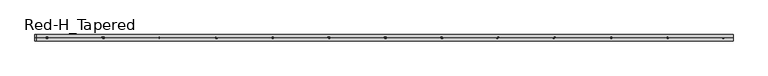
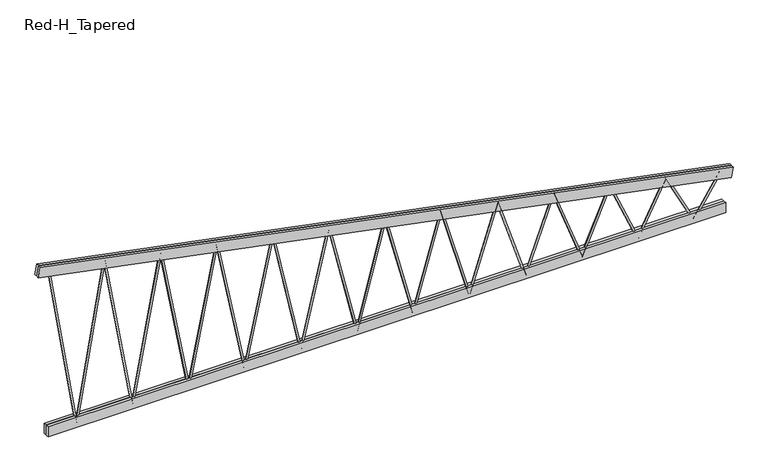
"""IFC4 building model written with IfcOpenShell, lengths in millimetres: beam geometry, Construction_Frames_RedBuilt_Openweb_Red-H_Tapered : Red-H_Tapered."""

import ifcopenshell
import ifcopenshell.guid

model = None  # the IFC model being written
_history = None  # IfcOwnerHistory: only IFC2X3 demands one
_inside = {}  # id of a spatial element -> (the spatial element, [elements in it])
_under = {}  # id of a project, library or spatial element -> (it, [spatial elements below it])
_declared = {}  # id of a project -> (the project, [libraries it declares])
_typed = {}  # id of a type object -> (the type object, [elements of that type])
_made_of = {}  # id of a material, layer set ... -> (it, [elements and type objects made of it])


def new_model(schema):
    """Start an empty IFC model of exactly this schema.

    Asked for "IFC4X3", IfcOpenShell would pick the latest addendum, in which some entities
    have other attributes; the version numbers below select the first issue.
    IFC2X3 requires an IfcOwnerHistory on every rooted entity: one is made here for all.
    """
    global model, _history
    if schema == "IFC4X3":
        model = ifcopenshell.file(schema_version=(4, 3, 0, 0))
    else:
        model = ifcopenshell.file(schema=schema)
    _inside.clear()
    _under.clear()
    _declared.clear()
    _typed.clear()
    _made_of.clear()
    _history = None
    if model.schema == "IFC2X3":
        org = make("IfcOrganization", Name="unknown")
        user = make(
            "IfcPersonAndOrganization",
            ThePerson=make("IfcPerson", FamilyName="unknown"),
            TheOrganization=org,
        )
        app = make(
            "IfcApplication",
            ApplicationDeveloper=org,
            Version="unknown",
            ApplicationFullName="unknown",
            ApplicationIdentifier="unknown",
        )
        _history = make(
            "IfcOwnerHistory",
            OwningUser=user,
            OwningApplication=app,
            ChangeAction="ADDED",
            CreationDate=0,
        )
    return model


def make(cls, **values):
    """One entity of the class cls with the attributes given. An attribute that is None is left unset."""
    return model.create_entity(
        cls, **{name: value for name, value in values.items() if value is not None}
    )


def rooted(cls, **values):
    """An entity with a GlobalId (a new one), such as an element, a storey or a relation."""
    return make(cls, GlobalId=ifcopenshell.guid.new(), OwnerHistory=_history, **values)


def si_unit(unit_type, name, prefix=None):
    """IfcSIUnit, for example si_unit("LENGTHUNIT", "METRE", prefix="MILLI")."""
    return make("IfcSIUnit", UnitType=unit_type, Prefix=prefix, Name=name)


def assignment(units):
    """IfcUnitAssignment: the units of a project."""
    return None if units is None else make("IfcUnitAssignment", Units=units)


def point(xyz):
    """IfcCartesianPoint."""
    return None if xyz is None else make("IfcCartesianPoint", Coordinates=xyz)


def direction(xyz):
    """IfcDirection."""
    return None if xyz is None else make("IfcDirection", DirectionRatios=xyz)


def frame(location, z_axis=None, x_axis=None):
    """IfcAxis2Placement3D, a coordinate frame: its origin and axes. An axis left out is left unset."""
    return make(
        "IfcAxis2Placement3D",
        Location=point(location),
        Axis=direction(z_axis),
        RefDirection=direction(x_axis),
    )


def frame_2d(location, x_axis=None):
    """IfcAxis2Placement2D, a coordinate frame in the plane: its origin and x axis."""
    return make(
        "IfcAxis2Placement2D", Location=point(location), RefDirection=direction(x_axis)
    )


def origin():
    """The frame at (0, 0, 0) with its axes left unset."""
    return frame((0.0, 0.0, 0.0))


def origin_2d():
    """The frame at (0, 0) in the plane with its x axis left unset."""
    return frame_2d((0.0, 0.0))


def place(relative_to, where):
    """IfcLocalPlacement: puts the frame where relative to a parent placement (None: the world)."""
    return make(
        "IfcLocalPlacement", PlacementRelTo=relative_to, RelativePlacement=where
    )


def context(
    kind, dimensions, precision=None, world=None, true_north=None, identifier=None
):
    """IfcGeometricRepresentationContext, for example the 3D "Model" context."""
    return make(
        "IfcGeometricRepresentationContext",
        ContextIdentifier=identifier,
        ContextType=kind,
        CoordinateSpaceDimension=dimensions,
        Precision=precision,
        WorldCoordinateSystem=world,
        TrueNorth=true_north,
    )


def project(units=None, contexts=None):
    """IfcProject with its units and contexts."""
    return rooted(
        "IfcProject",
        Name="project",
        RepresentationContexts=contexts,
        UnitsInContext=assignment(units),
    )


def spatial(cls, under=None, at=None, **own):
    """A site, building, storey or space (cls), placed at a placement, below another one or the project."""
    s = rooted(cls, ObjectPlacement=at, **own)
    if under is not None:
        _under.setdefault(under.id(), (under, []))[1].append(s)
    return s


def polyline(points):
    """IfcPolyline through the points."""
    return make("IfcPolyline", Points=[point(p) for p in points])


def circle_curve(where, radius):
    """IfcCircle in the frame where."""
    return make("IfcCircle", Position=where, Radius=radius)


def trimmed(basis, trim1, trim2, sense, master):
    """IfcTrimmedCurve: the piece of a basis curve between two trims."""
    return make(
        "IfcTrimmedCurve",
        BasisCurve=basis,
        Trim1=trim1,
        Trim2=trim2,
        SenseAgreement=sense,
        MasterRepresentation=master,
    )


def segment(curve, same_sense, transition):
    """IfcCompositeCurveSegment."""
    return make(
        "IfcCompositeCurveSegment",
        Transition=transition,
        SameSense=same_sense,
        ParentCurve=curve,
    )


def composite_curve(segments, self_intersect=None):
    """IfcCompositeCurve: segments joined end to end."""
    return make("IfcCompositeCurve", Segments=segments, SelfIntersect=self_intersect)


def outline(outer, holes=None, kind="AREA"):
    """IfcArbitraryClosedProfileDef: a profile drawn as a closed curve; with holes, ...WithVoids."""
    if holes is None:
        return make("IfcArbitraryClosedProfileDef", ProfileType=kind, OuterCurve=outer)
    return make(
        "IfcArbitraryProfileDefWithVoids",
        ProfileType=kind,
        OuterCurve=outer,
        InnerCurves=holes,
    )


def extrude(swept, where, along, depth):
    """IfcExtrudedAreaSolid: the profile swept, set in the frame where, extruded along a direction by depth."""
    return make(
        "IfcExtrudedAreaSolid",
        SweptArea=swept,
        Position=where,
        ExtrudedDirection=direction(along),
        Depth=depth,
    )


def shape(context_of_items, identifier, shape_type, items):
    """IfcShapeRepresentation: the items that make up one representation, for example the "Body"."""
    return make(
        "IfcShapeRepresentation",
        ContextOfItems=context_of_items,
        RepresentationIdentifier=identifier,
        RepresentationType=shape_type,
        Items=items,
    )


def source(mapping_origin, context_of_items, identifier, shape_type, items):
    """IfcRepresentationMap: a shape defined once, which mapped items show again and again."""
    return make(
        "IfcRepresentationMap",
        MappingOrigin=mapping_origin,
        MappedRepresentation=shape(context_of_items, identifier, shape_type, items),
    )


def transform(
    local_origin,
    x_axis=None,
    y_axis=None,
    z_axis=None,
    scale=None,
    scale2=None,
    scale3=None,
    uniform=True,
):
    """IfcCartesianTransformationOperator3D, or its non-uniform kind. x_axis, y_axis, z_axis: its Axis1, 2, 3."""
    if uniform:
        return make(
            "IfcCartesianTransformationOperator3D",
            Axis1=direction(x_axis),
            Axis2=direction(y_axis),
            LocalOrigin=point(local_origin),
            Scale=scale,
            Axis3=direction(z_axis),
        )
    return make(
        "IfcCartesianTransformationOperator3DnonUniform",
        Axis1=direction(x_axis),
        Axis2=direction(y_axis),
        LocalOrigin=point(local_origin),
        Scale=scale,
        Axis3=direction(z_axis),
        Scale2=scale2,
        Scale3=scale3,
    )


def mapped(mapping_source, mapping_target):
    """IfcMappedItem: shows the shape of a source again, moved by a transform."""
    return make(
        "IfcMappedItem", MappingSource=mapping_source, MappingTarget=mapping_target
    )


def made_of(thing, what):
    """Note that an element or type object is made of a material, layer set ...; save() writes the relation."""
    if what is not None:
        _made_of.setdefault(what.id(), (what, []))[1].append(thing)
    return thing


def element(
    cls,
    number,
    at=None,
    inside=None,
    cuts=None,
    type_object=None,
    material=None,
    context=None,
    identifier="Body",
    shape_type=None,
    held_by="IfcProductDefinitionShape",
    body=None,
    shapes=None,
    **own,
):
    """One element of the class cls, such as IfcWall. Its Tag is "e" and its number.

    at: its placement. inside: the storey or other place that contains it. cuts: it is an
    opening in that element (IfcRelVoidsElement). A single representation is given by context,
    identifier, shape_type and body (its items); several are given by shapes. held_by: the class
    of the entity that holds the representations. save() writes the other relations.
    """
    e = rooted(cls, Tag="e%d" % number, ObjectPlacement=at, **own)
    if body is not None:
        shapes = [shape(context, identifier, shape_type, body)]
    if shapes is not None:
        e.Representation = make(held_by, Representations=shapes)
    if inside is not None:
        _inside.setdefault(inside.id(), (inside, []))[1].append(e)
    if cuts is not None:
        rooted(
            "IfcRelVoidsElement", RelatingBuildingElement=cuts, RelatedOpeningElement=e
        )
    if type_object is not None:
        _typed.setdefault(type_object.id(), (type_object, []))[1].append(e)
    return made_of(e, material)


def aggregate(whole, parts):
    """IfcRelAggregates: a whole, such as a stair, and the parts it consists of."""
    return rooted("IfcRelAggregates", RelatingObject=whole, RelatedObjects=parts)


def save(model, path):
    """Write the relations noted so far, then the file.

    IfcRelAggregates (storeys below a building ...), IfcRelContainedInSpatialStructure (elements
    in a storey), IfcRelDefinesByType, IfcRelAssociatesMaterial and IfcRelDeclares: one each for
    every whole, place, type object, material and project.
    """
    for whole, parts in _under.values():
        aggregate(whole, parts)
    for where, things in _inside.values():
        rooted(
            "IfcRelContainedInSpatialStructure",
            RelatedElements=things,
            RelatingStructure=where,
        )
    for kind, things in _typed.values():
        rooted("IfcRelDefinesByType", RelatedObjects=things, RelatingType=kind)
    for what, things in _made_of.values():
        rooted("IfcRelAssociatesMaterial", RelatedObjects=things, RelatingMaterial=what)
    for by, libraries in _declared.values():
        rooted("IfcRelDeclares", RelatingContext=by, RelatedDefinitions=libraries)
    model.write(path)


def red_h_tapered_448002e5(model_context):
    return source(origin(), model_context, "Body", "SweptSolid", [
        extrude(outline(composite_curve([segment(trimmed(circle_curve(origin_2d(), 12.7), [point((0.0, 12.7))], [point((0.0, -12.7000001))], False, "CARTESIAN"), True, "CONTINUOUS"), segment(trimmed(circle_curve(origin_2d(), 12.7), [point((0.0, -12.7000001))], [point((0.0, 12.7))], False, "CARTESIAN"), True, "CONTINUOUS")], self_intersect=False)), frame((-4144.4333333, 0.0, -367.0101562), z_axis=(-0.1588441891295665, 0.0, 0.9873036633071766), x_axis=(0.0, -1.0, 0.0)), (0.0, 0.0, 1.0), 2371.9260285),
        extrude(outline(composite_curve([segment(trimmed(circle_curve(origin_2d(), 12.7), [point((0.0, -12.7))], [point((0.0, 12.7))], False, "CARTESIAN"), True, "CONTINUOUS"), segment(trimmed(circle_curve(origin_2d(), 12.7), [point((0.0, 12.7))], [point((0.0, -12.7))], False, "CARTESIAN"), True, "CONTINUOUS")], self_intersect=False)), frame((1130.3, 0.0, -367.0101562), z_axis=(-0.2751349261836707, 0.0, 0.9614056232381346), x_axis=(0.0, -1.0, 0.0)), (0.0, 0.0, 1.0), 1369.3887283),
        extrude(outline(composite_curve([segment(trimmed(circle_curve(origin_2d(), 12.7), [point((0.0, 12.7))], [point((0.0, -12.7))], False, "CARTESIAN"), True, "CONTINUOUS"), segment(trimmed(circle_curve(origin_2d(), 12.7), [point((0.0, -12.7))], [point((0.0, 12.7))], False, "CARTESIAN"), True, "CONTINUOUS")], self_intersect=False)), frame((376.7666667, 0.0, -367.0101562), z_axis=(0.2751349261836737, 0.0, 0.9614056232381338), x_axis=(0.0, -1.0, 0.0)), (0.0, 0.0, 1.0), 1369.3887283),
        extrude(outline(composite_curve([segment(trimmed(circle_curve(origin_2d(), 12.7), [point((0.0, -12.7))], [point((0.0, 12.7))], False, "CARTESIAN"), True, "CONTINUOUS"), segment(trimmed(circle_curve(origin_2d(), 12.7), [point((0.0, 12.7))], [point((0.0, -12.7))], False, "CARTESIAN"), True, "CONTINUOUS")], self_intersect=False)), frame((376.7666667, 0.0, -367.0101562), z_axis=(-0.24939195296979247, 0.0, 0.9684026300015469), x_axis=(0.0, -1.0, 0.0)), (0.0, 0.0, 1.0), 1510.7410732),
        extrude(outline(composite_curve([segment(trimmed(circle_curve(origin_2d(), 12.7), [point((0.0, 12.7))], [point((0.0, -12.7))], False, "CARTESIAN"), True, "CONTINUOUS"), segment(trimmed(circle_curve(origin_2d(), 12.7), [point((0.0, -12.7))], [point((0.0, 12.7))], False, "CARTESIAN"), True, "CONTINUOUS")], self_intersect=False)), frame((-376.7666667, 0.0, -367.0101562), z_axis=(0.24939195296976147, 0.0, 0.9684026300015548), x_axis=(0.0, -1.0, 0.0)), (0.0, 0.0, 1.0), 1510.7410732),
        extrude(outline(composite_curve([segment(trimmed(circle_curve(origin_2d(), 12.7), [point((0.0, -12.7))], [point((0.0, 12.7))], False, "CARTESIAN"), True, "CONTINUOUS"), segment(trimmed(circle_curve(origin_2d(), 12.7), [point((0.0, 12.7))], [point((0.0, -12.7))], False, "CARTESIAN"), True, "CONTINUOUS")], self_intersect=False)), frame((-376.7666667, 0.0, -367.0101562), z_axis=(-0.22793117807234023, 0.0, 0.9736772453244222), x_axis=(0.0, -1.0, 0.0)), (0.0, 0.0, 1.0), 1652.9843344),
        extrude(outline(composite_curve([segment(trimmed(circle_curve(origin_2d(), 12.7), [point((0.0, 12.7))], [point((0.0, -12.7))], False, "CARTESIAN"), True, "CONTINUOUS"), segment(trimmed(circle_curve(origin_2d(), 12.7), [point((0.0, -12.7))], [point((0.0, 12.7))], False, "CARTESIAN"), True, "CONTINUOUS")], self_intersect=False)), frame((-1130.3, 0.0, -367.0101562), z_axis=(0.22793117807234073, 0.0, 0.9736772453244221), x_axis=(0.0, -1.0, 0.0)), (0.0, 0.0, 1.0), 1652.9843344),
        extrude(outline(composite_curve([segment(trimmed(circle_curve(origin_2d(), 12.7), [point((0.0, -12.7))], [point((0.0, 12.7))], False, "CARTESIAN"), True, "CONTINUOUS"), segment(trimmed(circle_curve(origin_2d(), 12.7), [point((0.0, 12.7))], [point((0.0, -12.7))], False, "CARTESIAN"), True, "CONTINUOUS")], self_intersect=False)), frame((-1130.3, 0.0, -367.0101562), z_axis=(-0.20979187786626347, 0.0, 0.9777460651832596), x_axis=(0.0, -1.0, 0.0)), (0.0, 0.0, 1.0), 1795.9068316),
        extrude(outline(composite_curve([segment(trimmed(circle_curve(origin_2d(), 12.7), [point((0.0, -12.7000001))], [point((0.0, 12.7))], False, "CARTESIAN"), True, "CONTINUOUS"), segment(trimmed(circle_curve(origin_2d(), 12.7), [point((0.0, 12.7))], [point((0.0, -12.7000001))], False, "CARTESIAN"), True, "CONTINUOUS")], self_intersect=False)), frame((-1883.8333333, 0.0, -367.0101562), z_axis=(0.20979187786626646, 0.0, 0.9777460651832589), x_axis=(0.0, -1.0, 0.0)), (0.0, 0.0, 1.0), 1795.9068316),
        extrude(outline(composite_curve([segment(trimmed(circle_curve(origin_2d(), 12.7), [point((0.0, 12.6999999))], [point((0.0, -12.7))], False, "CARTESIAN"), True, "CONTINUOUS"), segment(trimmed(circle_curve(origin_2d(), 12.7), [point((0.0, -12.7))], [point((0.0, 12.6999999))], False, "CARTESIAN"), True, "CONTINUOUS")], self_intersect=False)), frame((-1883.8333333, 0.0, -367.0101562), z_axis=(-0.19427387255590262, 0.0, 0.9809473290865993), x_axis=(0.0, -1.0, 0.0)), (0.0, 0.0, 1.0), 1939.3584001),
        extrude(outline(composite_curve([segment(trimmed(circle_curve(origin_2d(), 12.7), [point((0.0, -12.6999999))], [point((0.0, 12.7))], False, "CARTESIAN"), True, "CONTINUOUS"), segment(trimmed(circle_curve(origin_2d(), 12.7), [point((0.0, 12.7))], [point((0.0, -12.6999999))], False, "CARTESIAN"), True, "CONTINUOUS")], self_intersect=False)), frame((-2637.3666667, 0.0, -367.0101562), z_axis=(0.19427387255590164, 0.0, 0.9809473290865995), x_axis=(0.0, -1.0, 0.0)), (0.0, 0.0, 1.0), 1939.3584001),
        extrude(outline(composite_curve([segment(trimmed(circle_curve(origin_2d(), 12.7), [point((0.0, 12.7000001))], [point((0.0, -12.7))], False, "CARTESIAN"), True, "CONTINUOUS"), segment(trimmed(circle_curve(origin_2d(), 12.7), [point((0.0, -12.7))], [point((0.0, 12.7000001))], False, "CARTESIAN"), True, "CONTINUOUS")], self_intersect=False)), frame((-2637.3666667, 0.0, -367.0101562), z_axis=(-0.180856992463189, 0.0, 0.983509404264733), x_axis=(0.0, -1.0, 0.0)), (0.0, 0.0, 1.0), 2083.2297471),
        extrude(outline(composite_curve([segment(trimmed(circle_curve(origin_2d(), 12.7), [point((0.0, -12.7))], [point((0.0, 12.7))], False, "CARTESIAN"), True, "CONTINUOUS"), segment(trimmed(circle_curve(origin_2d(), 12.7), [point((0.0, 12.7))], [point((0.0, -12.7))], False, "CARTESIAN"), True, "CONTINUOUS")], self_intersect=False)), frame((-3390.9, 0.0, -367.0101562), z_axis=(0.18085699246319326, 0.0, 0.9835094042647322), x_axis=(0.0, -1.0, 0.0)), (0.0, 0.0, 1.0), 2083.2297471),
        extrude(outline(composite_curve([segment(trimmed(circle_curve(origin_2d(), 12.7), [point((0.0, 12.7))], [point((0.0, -12.7))], False, "CARTESIAN"), True, "CONTINUOUS"), segment(trimmed(circle_curve(origin_2d(), 12.7), [point((0.0, -12.7))], [point((0.0, 12.7))], False, "CARTESIAN"), True, "CONTINUOUS")], self_intersect=False)), frame((-3390.9, 0.0, -367.0101562), z_axis=(-0.16914787634304293, 0.0, 0.9855906837671705), x_axis=(0.0, -1.0, 0.0)), (0.0, 0.0, 1.0), 2227.4395329),
        extrude(outline(composite_curve([segment(trimmed(circle_curve(origin_2d(), 12.7), [point((0.0, -12.7))], [point((0.0, 12.7))], False, "CARTESIAN"), True, "CONTINUOUS"), segment(trimmed(circle_curve(origin_2d(), 12.7), [point((0.0, 12.7))], [point((0.0, -12.7))], False, "CARTESIAN"), True, "CONTINUOUS")], self_intersect=False)), frame((-4144.4333333, 0.0, -367.0101562), z_axis=(0.16914787634304163, 0.0, 0.9855906837671707), x_axis=(0.0, -1.0, 0.0)), (0.0, 0.0, 1.0), 2227.4395329),
        extrude(outline(composite_curve([segment(trimmed(circle_curve(origin_2d(), 12.7), [point((0.0, 12.7))], [point((0.0, -12.7))], False, "CARTESIAN"), True, "CONTINUOUS"), segment(trimmed(circle_curve(origin_2d(), 12.7), [point((0.0, -12.7))], [point((0.0, 12.7))], False, "CARTESIAN"), True, "CONTINUOUS")], self_intersect=False)), frame((4144.4333333, 0.0, -367.0101562), z_axis=(0.5419881538462402, 0.0, 0.8403861261886374), x_axis=(0.0, -1.0, 0.0)), (0.0, 0.0, 1.0), 695.156645),
        extrude(outline(composite_curve([segment(trimmed(circle_curve(origin_2d(), 12.7), [point((0.0, -12.7))], [point((0.0, 12.7))], False, "CARTESIAN"), True, "CONTINUOUS"), segment(trimmed(circle_curve(origin_2d(), 12.7), [point((0.0, 12.7))], [point((0.0, -12.7))], False, "CARTESIAN"), True, "CONTINUOUS")], self_intersect=False)), frame((4144.4333333, 0.0, -367.0101562), z_axis=(-0.4583046838689422, 0.0, 0.8887951489200361), x_axis=(0.0, -1.0, 0.0)), (0.0, 0.0, 1.0), 822.0877506),
        extrude(outline(composite_curve([segment(trimmed(circle_curve(origin_2d(), 12.7), [point((0.0, 12.7))], [point((0.0, -12.7))], False, "CARTESIAN"), True, "CONTINUOUS"), segment(trimmed(circle_curve(origin_2d(), 12.7), [point((0.0, -12.7))], [point((0.0, 12.7))], False, "CARTESIAN"), True, "CONTINUOUS")], self_intersect=False)), frame((3390.9, 0.0, -367.0101562), z_axis=(0.45830468386894385, 0.0, 0.8887951489200352), x_axis=(0.0, -1.0, 0.0)), (0.0, 0.0, 1.0), 822.0877506),
        extrude(outline(composite_curve([segment(trimmed(circle_curve(origin_2d(), 12.7), [point((0.0, -12.7))], [point((0.0, 12.7))], False, "CARTESIAN"), True, "CONTINUOUS"), segment(trimmed(circle_curve(origin_2d(), 12.7), [point((0.0, 12.7))], [point((0.0, -12.7))], False, "CARTESIAN"), True, "CONTINUOUS")], self_intersect=False)), frame((3390.9, 0.0, -367.0101562), z_axis=(-0.3946727935442272, 0.0, 0.91882173789914), x_axis=(0.0, -1.0, 0.0)), (0.0, 0.0, 1.0), 954.6304504),
        extrude(outline(composite_curve([segment(trimmed(circle_curve(origin_2d(), 12.7), [point((0.0, 12.6999999))], [point((0.0, -12.7))], False, "CARTESIAN"), True, "CONTINUOUS"), segment(trimmed(circle_curve(origin_2d(), 12.7), [point((0.0, -12.7))], [point((0.0, 12.6999999))], False, "CARTESIAN"), True, "CONTINUOUS")], self_intersect=False)), frame((2637.3666667, 0.0, -367.0101562), z_axis=(0.3946727935442274, 0.0, 0.9188217378991399), x_axis=(0.0, -1.0, 0.0)), (0.0, 0.0, 1.0), 954.6304504),
        extrude(outline(composite_curve([segment(trimmed(circle_curve(origin_2d(), 12.7), [point((0.0, -12.7))], [point((0.0, 12.7))], False, "CARTESIAN"), True, "CONTINUOUS"), segment(trimmed(circle_curve(origin_2d(), 12.7), [point((0.0, 12.7))], [point((0.0, -12.7))], False, "CARTESIAN"), True, "CONTINUOUS")], self_intersect=False)), frame((2637.3666667, 0.0, -367.0101562), z_axis=(-0.3454226808968656, 0.0, 0.9384472129651311), x_axis=(0.0, -1.0, 0.0)), (0.0, 0.0, 1.0), 1090.7409603),
        extrude(outline(composite_curve([segment(trimmed(circle_curve(origin_2d(), 12.7), [point((0.0, 12.7))], [point((0.0, -12.7))], False, "CARTESIAN"), True, "CONTINUOUS"), segment(trimmed(circle_curve(origin_2d(), 12.7), [point((0.0, -12.7))], [point((0.0, 12.7))], False, "CARTESIAN"), True, "CONTINUOUS")], self_intersect=False)), frame((1883.8333333, 0.0, -367.0101562), z_axis=(0.345422680896868, 0.0, 0.9384472129651302), x_axis=(0.0, -1.0, 0.0)), (0.0, 0.0, 1.0), 1090.7409603),
        extrude(outline(composite_curve([segment(trimmed(circle_curve(origin_2d(), 12.7), [point((0.0, -12.7))], [point((0.0, 12.7))], False, "CARTESIAN"), True, "CONTINUOUS"), segment(trimmed(circle_curve(origin_2d(), 12.7), [point((0.0, 12.7))], [point((0.0, -12.7))], False, "CARTESIAN"), True, "CONTINUOUS")], self_intersect=False)), frame((1883.8333333, 0.0, -367.0101562), z_axis=(-0.30650507327676635, 0.0, 0.9518690246329082), x_axis=(0.0, -1.0, 0.0)), (0.0, 0.0, 1.0), 1229.2346833),
        extrude(outline(composite_curve([segment(trimmed(circle_curve(origin_2d(), 12.7), [point((0.0, 12.7))], [point((0.0, -12.7))], False, "CARTESIAN"), True, "CONTINUOUS"), segment(trimmed(circle_curve(origin_2d(), 12.7), [point((0.0, -12.7))], [point((0.0, 12.7))], False, "CARTESIAN"), True, "CONTINUOUS")], self_intersect=False)), frame((1130.3, 0.0, -367.0101562), z_axis=(0.3065050732767705, 0.0, 0.951869024632907), x_axis=(0.0, -1.0, 0.0)), (0.0, 0.0, 1.0), 1229.2346833),
        extrude(outline(polyline([(-4546.6, -41.275), (-4546.6, -3.175), (4546.6, -3.175), (4546.6, -41.275), (-4546.6, -41.275)])), frame((0.0, 0.0, -386.0601562), z_axis=(0.0, 0.0, 1.0), x_axis=(1.0, 0.0, 0.0)), (0.0, 0.0, 1.0), 139.7),
        extrude(outline(polyline([(-4546.6, 3.175), (-4546.6, 41.275), (4546.6, 41.275), (4546.6, 3.175), (-4546.6, 3.175)])), frame((0.0, 0.0, -386.0601562), z_axis=(0.0, 0.0, 1.0), x_axis=(1.0, 0.0, 0.0)), (0.0, 0.0, 1.0), 139.7),
        extrude(outline(polyline([(0.0, -38.1), (0.0, 0.0), (9474.5745234, 0.0), (9474.5745234, -38.1), (0.0, -38.1)])), frame((-4675.1651539, -3.175, 1915.2669782), z_axis=(0.19302186029333512, 0.0, 0.9811944564911179), x_axis=(0.9811944564911179, 0.0, -0.19302186029333512)), (0.0, 0.0, 1.0), 139.7),
        extrude(outline(polyline([(0.0, -38.1), (0.0, 0.0), (9474.5745234, 0.0), (9474.5745234, -38.1), (0.0, -38.1)])), frame((-4675.1651539, 41.275, 1915.2669782), z_axis=(0.19302186029333512, 0.0, 0.9811944564911179), x_axis=(0.9811944564911179, 0.0, -0.19302186029333512)), (0.0, 0.0, 1.0), 139.7),
    ])


if __name__ == "__main__":
    model = new_model("IFC4")
    model_context = context("Model", 3, world=origin())
    ifc_project = project(units=[si_unit("LENGTHUNIT", "METRE", prefix="MILLI")], contexts=[model_context])
    site = spatial("IfcSite", under=ifc_project)
    building = spatial("IfcBuilding", under=site)
    placement = place(None, origin())
    red_h_tapered_shape = red_h_tapered_448002e5(model_context)
    element("IfcBeam", 1, ObjectType="Construction_Frames_RedBuilt_Openweb_Red-H_Tapered : Red-H_Tapered", at=placement, inside=building, context=model_context, shape_type="MappedRepresentation", body=[
        mapped(red_h_tapered_shape, transform((0.0, 0.0, 0.0), x_axis=(1.0, 0.0, 0.0), y_axis=(0.0, 1.0, 0.0), z_axis=(0.0, 0.0, 1.0))),
    ])
    save(model, "model.ifc")

# Revit data of these elements
# Type "Construction_Frames_RedBuilt_Openweb_Red-H_Tapered : Red-H_Tapered"
#   Youtube clip = ""
#   Weight Net (Kg) = "0"
#   Webs = "Up to 2\" diameter tubular steel"
#   Uniformat II Description = ""
#   Uniformat II Code = ""
#   Uniclass 2015 Name = "Softwood trusses"
#   Uniclass 2015 Code = "Pr_20_85_90_81"
#   Uniclass 2.0 Description = "Structural Framing Systems"
#   Uniclass 2.0 Code = "SS-15-10-75"
#   Uniclass 1.4 Description = "Trusses"
#   Uniclass 1.4 Code = "L3523"
#   UNSPSC Code = "30103606"
#   Technical description = "http://www.redbuilt.com/reference/literature-and-other-resources"
#   Region South America = "None"
#   Region Oceania = "None"
#   Region North America = "US"
#   Region Middle East = "None"
#   Region Europe = "None"
#   Region Asia = "None"
#   Region Antarctica = "None"
#   Region Africa = "None"
#   QR code = "http://bimobject.com/redbuilt/product/redbuilt-0003"
#   Product url = "http://www.redbuilt.com/products/default.aspx?id=2"
#   Product group = "Wood Trusses"
#   Product family = "Construction"
#   Product data url = "https://bimobject.com/redbuilt/product/redbuilt-0003"
#   Product certification = ""
#   Product SKU = "redbuilt-0003"
#   Product Page URL = "http://www.redbuilt.com/commercial-systems/red-m-red-h-open-web-trusses"
#   Product Guid = "2c5793f2-6ffb-4665-b825-cf90c048e711"
#   Product Documentation Link = "http://www.redbuilt.com/documents/OW_Guide_2017_07_LowRes_wLinks.pdf"
#   OmniClass Description = "Wood Trusses"
#   OmniClass Code = "23-13 35 19 13 17"
#   NBS Reference Description = ""
#   NBS Reference Code = ""
#   Material secondary = "Steel"
#   Material main = "Wood"
#   Masterformat 2014 Description = "Metal-Web Wood Joists"
#   Masterformat 2014 Code = "06 17 36"
#   Manufacturer name = "RedBuilt"
#   Manufacturer country = "United States"
#   Installation instructions = "http://www.redbuilt.com/documents/Installation_Sheets_Open-Web.pdf"
#   IFC Classification = ""
#   EAN code = ""
#   Design country = "United States"
#   Product Information = "http://redbuilt.com/products/default.aspx?id=2"
#   Model = "Red-H-Tapered"
#   Manufacturer URL = "http://redbuilt.com/"
#   Manufacturer = "RedBuilt™"
#   Description = "Open Web Truss"
#   Date of publishing = "8/17/2010"
#   Contact us = "http://redbuilt.com/contact/"
#   Chords = "Double 1½\" x 5½\" MSR lumber"
#   COBIe Type Category = ""
#   Brand url = "http://www.redbuilt.com"
#   BIMobject main category code = "construction"
#   BIMobject main category = "Construction"
#   BIMobject category code = "construction-frames-trusses"
#   BIMobject category = "Frames & Trusses"
#   Web Radius = 0' - 0 1/2"
#   Web Layout Offset Start [instance default] = 0' - 5"
#   Web Layout Offset End [instance default] = 0' - 5"
#   Web Diameter = 0' - 1"
#   TotalLength [instance default] = 20' - 0"
#   Span Minimum = 4' - 0"
#   Span Maximum = 70' - 0"
#   Span Limit [instance default] = 20' - 0"
#   Nominal width = 0' - 0"
#   Nominal height = 0' - 0"
#   Inner Depth Top [instance default] = 0' - 2.76372"
#   Depth Start [instance default] = 6' - 0"
#   Top Chord Length [instance default] = 20' - 1.19701"
#   TC Extension Start Aux [instance default] = 0' - 0"
#   TC Extension End Aux [instance default] = 0' - 0"
#   T-B Chord Length Difference L [instance default] = 0' - 4"
#   T-B Chord Length Difference [instance default] = 0' - 4"
#   Height 2 [instance default] = 6' - 0"
#   Depth Minimum at Wall = 2' - 0"
#   Depth Maximum at Wall = 6' - 0"
#   Depth Lower End [instance default] = 2' - 0"
#   Depth Higher End [instance default] = 6' - 0"
#   Depth End [instance default] = 2' - 0"
#   Depth 2 [instance default] = 2' - 0"
#   Chord Width = 0' - 3 1/4"
#   Chord Thickness = 0' - 1 1/2"
#   Chord Depth = 0' - 5 1/2"
#   Offset Start [instance default] = 0' - 0"
#   TC Extension Start [instance default] = 0' - 0"
#   End Panel = 0' - 5"
#   Offset End [instance default] = 0' - 0"
#   TC Extension End [instance default] = 0' - 0"
#   Length [instance default] = 20' - 0"
#   Angle [instance default] = 5.71059°
#   Span Limit Warning [instance default] = no
#   Edition number = 1
#   Top Bearing Start [instance default] = yes
#   Top Bearing End [instance default] = yes
#   Bottom Bearing Start [instance default] = no
#   Bottom Bearing End [instance default] = no
#   8 Panels [instance default] = yes
#   16 Panels [instance default] = no
#   12 Panels [instance default] = no
#   Web Material = RedBuilt-Steel, Galvanized
#   Clip Material = RedBuilt-Steel, Galvanized
#   Chords Material = RedBuilt-MSR
#   URL = ""
#   Assembly Code = ""
# Element 1 (IfcBeam, "Construction_Frames_RedBuilt_Openweb_Red-H_Tapered : Red-H_Tapered")
#   TotalLength = 30' - 6"
#   Span Limit = 30' - 6"
#   Inner Depth Top = 0' - 2.80271"
#   Top Chord Length = 31' - 1.01475"
#   Depth 2 = 6' - 0"
#   Angle = 11.1292°
#   8 Panels = no
#   12 Panels = yes
#   Materials on its faces: "RedBuilt-Steel, Galvanized", "RedBuilt-MSR"
# Materials
#   "RedBuilt-Steel, Galvanized": class "Metal", colour RGB 164 172 176, transparency 0, Manufacturer = "RedBuilt. LLC", Comments = "Openweb Metal Web", URL = "http://www.redbuilt.com/", Description = "Galvanized steel", Cost = 0
#   "RedBuilt-MSR": class "Wood", colour RGB 213 182 136, transparency 0, Manufacturer = "RedBuilt, LLC", URL = "http://www.redbuilt.com/", Cost = 0
